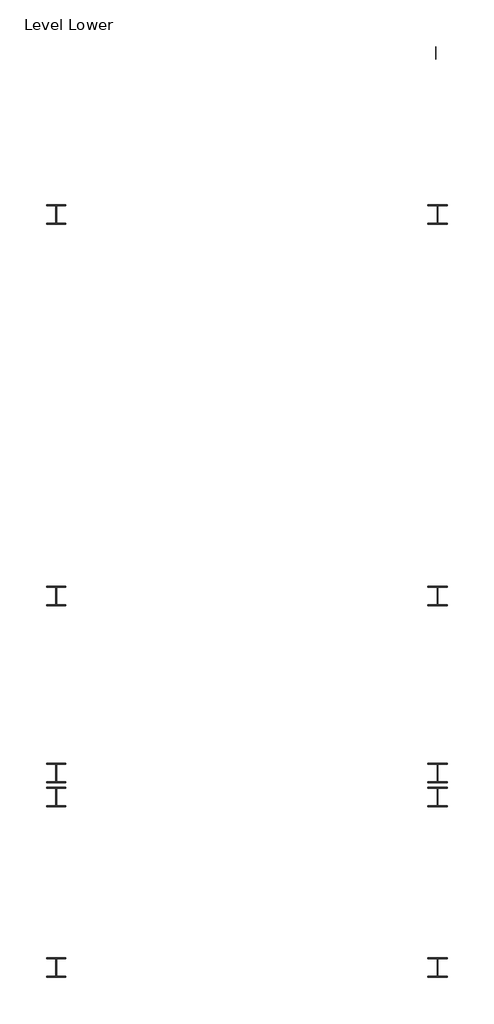
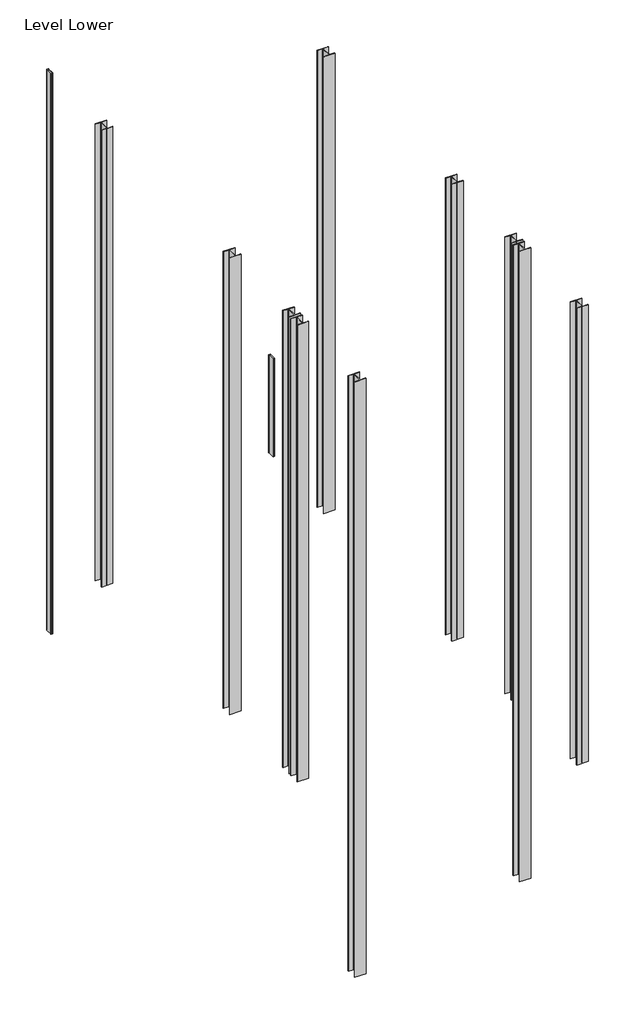
# One storey: 12 columns.
"""IFC4 building model written with IfcOpenShell, lengths in millimetres."""

import ifcopenshell
import ifcopenshell.guid

model = None  # the IFC model being written
_history = None  # IfcOwnerHistory: only IFC2X3 demands one
_inside = {}  # id of a spatial element -> (the spatial element, [elements in it])
_under = {}  # id of a project, library or spatial element -> (it, [spatial elements below it])
_declared = {}  # id of a project -> (the project, [libraries it declares])
_typed = {}  # id of a type object -> (the type object, [elements of that type])
_made_of = {}  # id of a material, layer set ... -> (it, [elements and type objects made of it])


def new_model(schema):
    """Start an empty IFC model of exactly this schema.

    Asked for "IFC4X3", IfcOpenShell would pick the latest addendum, in which some entities
    have other attributes; the version numbers below select the first issue.
    IFC2X3 requires an IfcOwnerHistory on every rooted entity: one is made here for all.
    """
    global model, _history
    if schema == "IFC4X3":
        model = ifcopenshell.file(schema_version=(4, 3, 0, 0))
    else:
        model = ifcopenshell.file(schema=schema)
    _inside.clear()
    _under.clear()
    _declared.clear()
    _typed.clear()
    _made_of.clear()
    _history = None
    if model.schema == "IFC2X3":
        org = make("IfcOrganization", Name="unknown")
        user = make(
            "IfcPersonAndOrganization",
            ThePerson=make("IfcPerson", FamilyName="unknown"),
            TheOrganization=org,
        )
        app = make(
            "IfcApplication",
            ApplicationDeveloper=org,
            Version="unknown",
            ApplicationFullName="unknown",
            ApplicationIdentifier="unknown",
        )
        _history = make(
            "IfcOwnerHistory",
            OwningUser=user,
            OwningApplication=app,
            ChangeAction="ADDED",
            CreationDate=0,
        )
    return model


def make(cls, **values):
    """One entity of the class cls with the attributes given. An attribute that is None is left unset."""
    return model.create_entity(
        cls, **{name: value for name, value in values.items() if value is not None}
    )


def rooted(cls, **values):
    """An entity with a GlobalId (a new one), such as an element, a storey or a relation."""
    return make(cls, GlobalId=ifcopenshell.guid.new(), OwnerHistory=_history, **values)


def si_unit(unit_type, name, prefix=None):
    """IfcSIUnit, for example si_unit("LENGTHUNIT", "METRE", prefix="MILLI")."""
    return make("IfcSIUnit", UnitType=unit_type, Prefix=prefix, Name=name)


def assignment(units):
    """IfcUnitAssignment: the units of a project."""
    return None if units is None else make("IfcUnitAssignment", Units=units)


def point(xyz):
    """IfcCartesianPoint."""
    return None if xyz is None else make("IfcCartesianPoint", Coordinates=xyz)


def direction(xyz):
    """IfcDirection."""
    return None if xyz is None else make("IfcDirection", DirectionRatios=xyz)


def frame(location, z_axis=None, x_axis=None):
    """IfcAxis2Placement3D, a coordinate frame: its origin and axes. An axis left out is left unset."""
    return make(
        "IfcAxis2Placement3D",
        Location=point(location),
        Axis=direction(z_axis),
        RefDirection=direction(x_axis),
    )


def frame_2d(location, x_axis=None):
    """IfcAxis2Placement2D, a coordinate frame in the plane: its origin and x axis."""
    return make(
        "IfcAxis2Placement2D", Location=point(location), RefDirection=direction(x_axis)
    )


def origin():
    """The frame at (0, 0, 0) with its axes left unset."""
    return frame((0.0, 0.0, 0.0))


def place(relative_to, where):
    """IfcLocalPlacement: puts the frame where relative to a parent placement (None: the world)."""
    return make(
        "IfcLocalPlacement", PlacementRelTo=relative_to, RelativePlacement=where
    )


def context(
    kind, dimensions, precision=None, world=None, true_north=None, identifier=None
):
    """IfcGeometricRepresentationContext, for example the 3D "Model" context."""
    return make(
        "IfcGeometricRepresentationContext",
        ContextIdentifier=identifier,
        ContextType=kind,
        CoordinateSpaceDimension=dimensions,
        Precision=precision,
        WorldCoordinateSystem=world,
        TrueNorth=true_north,
    )


def project(units=None, contexts=None):
    """IfcProject with its units and contexts."""
    return rooted(
        "IfcProject",
        Name="project",
        RepresentationContexts=contexts,
        UnitsInContext=assignment(units),
    )


def spatial(cls, under=None, at=None, **own):
    """A site, building, storey or space (cls), placed at a placement, below another one or the project."""
    s = rooted(cls, ObjectPlacement=at, **own)
    if under is not None:
        _under.setdefault(under.id(), (under, []))[1].append(s)
    return s


def polyline(points):
    """IfcPolyline through the points."""
    return make("IfcPolyline", Points=[point(p) for p in points])


def circle_curve(where, radius):
    """IfcCircle in the frame where."""
    return make("IfcCircle", Position=where, Radius=radius)


def trimmed(basis, trim1, trim2, sense, master):
    """IfcTrimmedCurve: the piece of a basis curve between two trims."""
    return make(
        "IfcTrimmedCurve",
        BasisCurve=basis,
        Trim1=trim1,
        Trim2=trim2,
        SenseAgreement=sense,
        MasterRepresentation=master,
    )


def segment(curve, same_sense, transition):
    """IfcCompositeCurveSegment."""
    return make(
        "IfcCompositeCurveSegment",
        Transition=transition,
        SameSense=same_sense,
        ParentCurve=curve,
    )


def composite_curve(segments, self_intersect=None):
    """IfcCompositeCurve: segments joined end to end."""
    return make("IfcCompositeCurve", Segments=segments, SelfIntersect=self_intersect)


def outline(outer, holes=None, kind="AREA"):
    """IfcArbitraryClosedProfileDef: a profile drawn as a closed curve; with holes, ...WithVoids."""
    if holes is None:
        return make("IfcArbitraryClosedProfileDef", ProfileType=kind, OuterCurve=outer)
    return make(
        "IfcArbitraryProfileDefWithVoids",
        ProfileType=kind,
        OuterCurve=outer,
        InnerCurves=holes,
    )


def extrude(swept, where, along, depth):
    """IfcExtrudedAreaSolid: the profile swept, set in the frame where, extruded along a direction by depth."""
    return make(
        "IfcExtrudedAreaSolid",
        SweptArea=swept,
        Position=where,
        ExtrudedDirection=direction(along),
        Depth=depth,
    )


def shape(context_of_items, identifier, shape_type, items):
    """IfcShapeRepresentation: the items that make up one representation, for example the "Body"."""
    return make(
        "IfcShapeRepresentation",
        ContextOfItems=context_of_items,
        RepresentationIdentifier=identifier,
        RepresentationType=shape_type,
        Items=items,
    )


def source(mapping_origin, context_of_items, identifier, shape_type, items):
    """IfcRepresentationMap: a shape defined once, which mapped items show again and again."""
    return make(
        "IfcRepresentationMap",
        MappingOrigin=mapping_origin,
        MappedRepresentation=shape(context_of_items, identifier, shape_type, items),
    )


def transform(
    local_origin,
    x_axis=None,
    y_axis=None,
    z_axis=None,
    scale=None,
    scale2=None,
    scale3=None,
    uniform=True,
):
    """IfcCartesianTransformationOperator3D, or its non-uniform kind. x_axis, y_axis, z_axis: its Axis1, 2, 3."""
    if uniform:
        return make(
            "IfcCartesianTransformationOperator3D",
            Axis1=direction(x_axis),
            Axis2=direction(y_axis),
            LocalOrigin=point(local_origin),
            Scale=scale,
            Axis3=direction(z_axis),
        )
    return make(
        "IfcCartesianTransformationOperator3DnonUniform",
        Axis1=direction(x_axis),
        Axis2=direction(y_axis),
        LocalOrigin=point(local_origin),
        Scale=scale,
        Axis3=direction(z_axis),
        Scale2=scale2,
        Scale3=scale3,
    )


def mapped(mapping_source, mapping_target):
    """IfcMappedItem: shows the shape of a source again, moved by a transform."""
    return make(
        "IfcMappedItem", MappingSource=mapping_source, MappingTarget=mapping_target
    )


def made_of(thing, what):
    """Note that an element or type object is made of a material, layer set ...; save() writes the relation."""
    if what is not None:
        _made_of.setdefault(what.id(), (what, []))[1].append(thing)
    return thing


def element(
    cls,
    number,
    at=None,
    inside=None,
    cuts=None,
    type_object=None,
    material=None,
    context=None,
    identifier="Body",
    shape_type=None,
    held_by="IfcProductDefinitionShape",
    body=None,
    shapes=None,
    **own,
):
    """One element of the class cls, such as IfcWall. Its Tag is "e" and its number.

    at: its placement. inside: the storey or other place that contains it. cuts: it is an
    opening in that element (IfcRelVoidsElement). A single representation is given by context,
    identifier, shape_type and body (its items); several are given by shapes. held_by: the class
    of the entity that holds the representations. save() writes the other relations.
    """
    e = rooted(cls, Tag="e%d" % number, ObjectPlacement=at, **own)
    if body is not None:
        shapes = [shape(context, identifier, shape_type, body)]
    if shapes is not None:
        e.Representation = make(held_by, Representations=shapes)
    if inside is not None:
        _inside.setdefault(inside.id(), (inside, []))[1].append(e)
    if cuts is not None:
        rooted(
            "IfcRelVoidsElement", RelatingBuildingElement=cuts, RelatedOpeningElement=e
        )
    if type_object is not None:
        _typed.setdefault(type_object.id(), (type_object, []))[1].append(e)
    return made_of(e, material)


def aggregate(whole, parts):
    """IfcRelAggregates: a whole, such as a stair, and the parts it consists of."""
    return rooted("IfcRelAggregates", RelatingObject=whole, RelatedObjects=parts)


def save(model, path):
    """Write the relations noted so far, then the file.

    IfcRelAggregates (storeys below a building ...), IfcRelContainedInSpatialStructure (elements
    in a storey), IfcRelDefinesByType, IfcRelAssociatesMaterial and IfcRelDeclares: one each for
    every whole, place, type object, material and project.
    """
    for whole, parts in _under.values():
        aggregate(whole, parts)
    for where, things in _inside.values():
        rooted(
            "IfcRelContainedInSpatialStructure",
            RelatedElements=things,
            RelatingStructure=where,
        )
    for kind, things in _typed.values():
        rooted("IfcRelDefinesByType", RelatedObjects=things, RelatingType=kind)
    for what, things in _made_of.values():
        rooted("IfcRelAssociatesMaterial", RelatedObjects=things, RelatingMaterial=what)
    for by, libraries in _declared.values():
        rooted("IfcRelDeclares", RelatingContext=by, RelatedDefinitions=libraries)
    model.write(path)


def hss_hollow_structural_section_column_hss8x2x3_16_e82f30fd(model_context):
    return source(origin(), model_context, "Body", "SweptSolid", [
        extrude(outline(composite_curve([segment(trimmed(circle_curve(frame_2d((16.5608, 92.7608)), 8.8392), [point((16.5608, 101.6))], [point((25.4, 92.7608))], False, "CARTESIAN"), True, "CONTINUOUS"), segment(polyline([(25.4, 92.7608), (25.4, -92.7608)]), True, "CONTINUOUS"), segment(trimmed(circle_curve(frame_2d((16.5608, -92.7608)), 8.8392), [point((25.4, -92.7608))], [point((16.5608, -101.6))], False, "CARTESIAN"), True, "CONTINUOUS"), segment(polyline([(16.5608, -101.6), (-16.5608, -101.6)]), True, "CONTINUOUS"), segment(trimmed(circle_curve(frame_2d((-16.5608, -92.7608)), 8.8392), [point((-16.5608, -101.6))], [point((-25.4, -92.7608))], False, "CARTESIAN"), True, "CONTINUOUS"), segment(polyline([(-25.4, -92.7608), (-25.4, 92.7608)]), True, "CONTINUOUS"), segment(trimmed(circle_curve(frame_2d((-16.5608, 92.7608)), 8.8392), [point((-25.4, 92.7608))], [point((-16.5608, 101.6))], False, "CARTESIAN"), True, "CONTINUOUS"), segment(polyline([(-16.5608, 101.6), (16.5608, 101.6)]), True, "CONTINUOUS")], self_intersect=False), holes=[composite_curve([segment(polyline([(16.5608, 97.1804), (-16.5608, 97.1804)]), True, "CONTINUOUS"), segment(trimmed(circle_curve(frame_2d((-16.5608, 92.7608)), 4.4196), [point((-16.5608, 97.1804))], [point((-20.9804, 92.7608))], True, "CARTESIAN"), True, "CONTINUOUS"), segment(polyline([(-20.9804, 92.7608), (-20.9804, -92.7608)]), True, "CONTINUOUS"), segment(trimmed(circle_curve(frame_2d((-16.5608, -92.7608)), 4.4196), [point((-20.9804, -92.7608))], [point((-16.5608, -97.1804))], True, "CARTESIAN"), True, "CONTINUOUS"), segment(polyline([(-16.5608, -97.1804), (16.5608, -97.1804)]), True, "CONTINUOUS"), segment(trimmed(circle_curve(frame_2d((16.5608, -92.7608)), 4.4196), [point((16.5608, -97.1804))], [point((20.9804, -92.7608))], True, "CARTESIAN"), True, "CONTINUOUS"), segment(polyline([(20.9804, -92.7608), (20.9804, 92.7608)]), True, "CONTINUOUS"), segment(trimmed(circle_curve(frame_2d((16.5608, 92.7608)), 4.4196), [point((20.9804, 92.7608))], [point((16.5608, 97.1804))], True, "CARTESIAN"), True, "CONTINUOUS")], self_intersect=False)]), frame((0.0, 0.0, -594.0), z_axis=(0.0, 0.0, 1.0), x_axis=(1.0, 0.0, 0.0)), (0.0, 0.0, 1.0), 2793.0),
    ])


def hss_hollow_structural_section_column_hss8x2x3_16_37e330f9(model_context):
    return source(origin(), model_context, "Body", "SweptSolid", [
        extrude(outline(composite_curve([segment(trimmed(circle_curve(frame_2d((16.5608, 92.7608)), 8.8392), [point((16.5608, 101.6))], [point((25.4, 92.7608))], False, "CARTESIAN"), True, "CONTINUOUS"), segment(polyline([(25.4, 92.7608), (25.4, -92.7608)]), True, "CONTINUOUS"), segment(trimmed(circle_curve(frame_2d((16.5608, -92.7608)), 8.8392), [point((25.4, -92.7608))], [point((16.5608, -101.6))], False, "CARTESIAN"), True, "CONTINUOUS"), segment(polyline([(16.5608, -101.6), (-16.5608, -101.6)]), True, "CONTINUOUS"), segment(trimmed(circle_curve(frame_2d((-16.5608, -92.7608)), 8.8392), [point((-16.5608, -101.6))], [point((-25.4, -92.7608))], False, "CARTESIAN"), True, "CONTINUOUS"), segment(polyline([(-25.4, -92.7608), (-25.4, 92.7608)]), True, "CONTINUOUS"), segment(trimmed(circle_curve(frame_2d((-16.5608, 92.7608)), 8.8392), [point((-25.4, 92.7608))], [point((-16.5608, 101.6))], False, "CARTESIAN"), True, "CONTINUOUS"), segment(polyline([(-16.5608, 101.6), (16.5608, 101.6)]), True, "CONTINUOUS")], self_intersect=False), holes=[composite_curve([segment(polyline([(16.5608, 97.1804), (-16.5608, 97.1804)]), True, "CONTINUOUS"), segment(trimmed(circle_curve(frame_2d((-16.5608, 92.7608)), 4.4196), [point((-16.5608, 97.1804))], [point((-20.9804, 92.7608))], True, "CARTESIAN"), True, "CONTINUOUS"), segment(polyline([(-20.9804, 92.7608), (-20.9804, -92.7608)]), True, "CONTINUOUS"), segment(trimmed(circle_curve(frame_2d((-16.5608, -92.7608)), 4.4196), [point((-20.9804, -92.7608))], [point((-16.5608, -97.1804))], True, "CARTESIAN"), True, "CONTINUOUS"), segment(polyline([(-16.5608, -97.1804), (16.5608, -97.1804)]), True, "CONTINUOUS"), segment(trimmed(circle_curve(frame_2d((16.5608, -92.7608)), 4.4196), [point((16.5608, -97.1804))], [point((20.9804, -92.7608))], True, "CARTESIAN"), True, "CONTINUOUS"), segment(polyline([(20.9804, -92.7608), (20.9804, 92.7608)]), True, "CONTINUOUS"), segment(trimmed(circle_curve(frame_2d((16.5608, 92.7608)), 4.4196), [point((20.9804, 92.7608))], [point((16.5608, 97.1804))], True, "CARTESIAN"), True, "CONTINUOUS")], self_intersect=False)]), frame((0.0, 0.0, -3550.0), z_axis=(0.0, 0.0, 1.0), x_axis=(1.0, 0.0, 0.0)), (0.0, 0.0, 1.0), 15989.0),
    ])


def uc_universal_columns_column_uc305x305x97_fcd1f718(model_context):
    return source(origin(), model_context, "Body", "SweptSolid", [
        extrude(outline(composite_curve([segment(polyline([(152.65, 153.95), (152.65, 138.55), (20.15, 138.55)]), True, "CONTINUOUS"), segment(trimmed(circle_curve(frame_2d((20.15, 123.35)), 15.2), [point((20.15, 138.55))], [point((4.95, 123.35))], True, "CARTESIAN"), True, "CONTINUOUS"), segment(polyline([(4.95, 123.35), (4.95, -123.35)]), True, "CONTINUOUS"), segment(trimmed(circle_curve(frame_2d((20.15, -123.35)), 15.2), [point((4.95, -123.35))], [point((20.15, -138.55))], True, "CARTESIAN"), True, "CONTINUOUS"), segment(polyline([(20.15, -138.55), (152.65, -138.55), (152.65, -153.95), (-152.65, -153.95), (-152.65, -138.55), (-20.15, -138.55)]), True, "CONTINUOUS"), segment(trimmed(circle_curve(frame_2d((-20.15, -123.35)), 15.2), [point((-20.15, -138.55))], [point((-4.95, -123.35))], True, "CARTESIAN"), True, "CONTINUOUS"), segment(polyline([(-4.95, -123.35), (-4.95, 123.35)]), True, "CONTINUOUS"), segment(trimmed(circle_curve(frame_2d((-20.15, 123.35)), 15.2), [point((-4.95, 123.35))], [point((-20.15, 138.55))], True, "CARTESIAN"), True, "CONTINUOUS"), segment(polyline([(-20.15, 138.55), (-152.65, 138.55), (-152.65, 153.95), (152.65, 153.95)]), True, "CONTINUOUS")], self_intersect=False)), frame((0.0, 0.0, -594.0), z_axis=(0.0, 0.0, 1.0), x_axis=(1.0, 0.0, 0.0)), (0.0, 0.0, 1.0), 13033.0),
    ])


def uc_universal_columns_column_uc305x305x97_02d5a26a(model_context):
    return source(origin(), model_context, "Body", "SweptSolid", [
        extrude(outline(composite_curve([segment(polyline([(152.65, 153.95), (152.65, 138.55), (20.15, 138.55)]), True, "CONTINUOUS"), segment(trimmed(circle_curve(frame_2d((20.15, 123.35)), 15.2), [point((20.15, 138.55))], [point((4.95, 123.35))], True, "CARTESIAN"), True, "CONTINUOUS"), segment(polyline([(4.95, 123.35), (4.95, -123.35)]), True, "CONTINUOUS"), segment(trimmed(circle_curve(frame_2d((20.15, -123.35)), 15.2), [point((4.95, -123.35))], [point((20.15, -138.55))], True, "CARTESIAN"), True, "CONTINUOUS"), segment(polyline([(20.15, -138.55), (152.65, -138.55), (152.65, -153.95), (-152.65, -153.95), (-152.65, -138.55), (-20.15, -138.55)]), True, "CONTINUOUS"), segment(trimmed(circle_curve(frame_2d((-20.15, -123.35)), 15.2), [point((-20.15, -138.55))], [point((-4.95, -123.35))], True, "CARTESIAN"), True, "CONTINUOUS"), segment(polyline([(-4.95, -123.35), (-4.95, 123.35)]), True, "CONTINUOUS"), segment(trimmed(circle_curve(frame_2d((-20.15, 123.35)), 15.2), [point((-4.95, 123.35))], [point((-20.15, 138.55))], True, "CARTESIAN"), True, "CONTINUOUS"), segment(polyline([(-20.15, 138.55), (-152.65, 138.55), (-152.65, 153.95), (152.65, 153.95)]), True, "CONTINUOUS")], self_intersect=False)), frame((0.0, 0.0, -4550.0), z_axis=(0.0, 0.0, 1.0), x_axis=(1.0, 0.0, 0.0)), (0.0, 0.0, 1.0), 16989.0),
    ])


def uc_universal_columns_column_uc305x305x97_e2fb10fc(model_context):
    return source(origin(), model_context, "Body", "SweptSolid", [
        extrude(outline(composite_curve([segment(polyline([(152.65, 153.95), (152.65, 138.55), (20.15, 138.55)]), True, "CONTINUOUS"), segment(trimmed(circle_curve(frame_2d((20.15, 123.35)), 15.2), [point((20.15, 138.55))], [point((4.95, 123.35))], True, "CARTESIAN"), True, "CONTINUOUS"), segment(polyline([(4.95, 123.35), (4.95, -123.35)]), True, "CONTINUOUS"), segment(trimmed(circle_curve(frame_2d((20.15, -123.35)), 15.2), [point((4.95, -123.35))], [point((20.15, -138.55))], True, "CARTESIAN"), True, "CONTINUOUS"), segment(polyline([(20.15, -138.55), (152.65, -138.55), (152.65, -153.95), (-152.65, -153.95), (-152.65, -138.55), (-20.15, -138.55)]), True, "CONTINUOUS"), segment(trimmed(circle_curve(frame_2d((-20.15, -123.35)), 15.2), [point((-20.15, -138.55))], [point((-4.95, -123.35))], True, "CARTESIAN"), True, "CONTINUOUS"), segment(polyline([(-4.95, -123.35), (-4.95, 123.35)]), True, "CONTINUOUS"), segment(trimmed(circle_curve(frame_2d((-20.15, 123.35)), 15.2), [point((-4.95, 123.35))], [point((-20.15, 138.55))], True, "CARTESIAN"), True, "CONTINUOUS"), segment(polyline([(-20.15, 138.55), (-152.65, 138.55), (-152.65, 153.95), (152.65, 153.95)]), True, "CONTINUOUS")], self_intersect=False)), frame((0.0, 0.0, -5550.0), z_axis=(0.0, 0.0, 1.0), x_axis=(1.0, 0.0, 0.0)), (0.0, 0.0, 1.0), 17989.0),
    ])


model = new_model("IFC4")

# Units and contexts
model_context = context("Model", 3, world=origin())
ifc_project = project(units=[si_unit("LENGTHUNIT", "METRE", prefix="MILLI")], contexts=[model_context])

# Site, building, storey
site = spatial("IfcSite", under=ifc_project)
building = spatial("IfcBuilding", under=site)
storey = spatial("IfcBuildingStorey", under=building, Name="Level Lower", Elevation=-550.0)

# Columns
placement = place(None, origin())
hss_hollow_structural_section_column_hss8x2x3_16_shape = hss_hollow_structural_section_column_hss8x2x3_16_e82f30fd(model_context)
element("IfcColumn", 1, ObjectType="HSS-Hollow Structural Section-Column : HSS8X2X3/16", at=placement, inside=storey, context=model_context, shape_type="MappedRepresentation", body=[
    mapped(hss_hollow_structural_section_column_hss8x2x3_16_shape, transform((13061.9315174, -3661.5939786, 0.0), x_axis=(1.0, 0.0, 0.0), y_axis=(0.0, 1.0, 0.0), z_axis=(0.0, 0.0, 1.0))),
])
hss_hollow_structural_section_column_hss8x2x3_16_2_shape = hss_hollow_structural_section_column_hss8x2x3_16_37e330f9(model_context)
element("IfcColumn", 2, ObjectType="HSS-Hollow Structural Section-Column : HSS8X2X3/16", at=placement, inside=storey, context=model_context, shape_type="MappedRepresentation", body=[
    mapped(hss_hollow_structural_section_column_hss8x2x3_16_2_shape, transform((7061.9315174, -3661.5939786, 0.0), x_axis=(1.0, 0.0, 0.0), y_axis=(0.0, 1.0, 0.0), z_axis=(0.0, 0.0, 1.0))),
])
uc_universal_columns_column_uc305x305x97_shape = uc_universal_columns_column_uc305x305x97_fcd1f718(model_context)
element("IfcColumn", 3, ObjectType="UC-Universal Columns-Column : UC305x305x97", at=placement, inside=storey, context=model_context, shape_type="MappedRepresentation", body=[
    mapped(uc_universal_columns_column_uc305x305x97_shape, transform((7061.9315174, -15361.5939786, 0.0), x_axis=(1.0, 0.0, 0.0), y_axis=(0.0, 1.0, 0.0), z_axis=(0.0, 0.0, 1.0))),
])
element("IfcColumn", 4, ObjectType="UC-Universal Columns-Column : UC305x305x97", at=placement, inside=storey, context=model_context, shape_type="MappedRepresentation", body=[
    mapped(uc_universal_columns_column_uc305x305x97_shape, transform((7061.9315174, -14981.5939786, 0.0), x_axis=(1.0, 0.0, 0.0), y_axis=(0.0, 1.0, 0.0), z_axis=(0.0, 0.0, 1.0))),
])
element("IfcColumn", 5, ObjectType="UC-Universal Columns-Column : UC305x305x97", at=placement, inside=storey, context=model_context, shape_type="MappedRepresentation", body=[
    mapped(uc_universal_columns_column_uc305x305x97_shape, transform((7061.9315174, -12201.5939786, 0.0), x_axis=(1.0, 0.0, 0.0), y_axis=(0.0, 1.0, 0.0), z_axis=(0.0, 0.0, 1.0))),
])
element("IfcColumn", 6, ObjectType="UC-Universal Columns-Column : UC305x305x97", at=placement, inside=storey, context=model_context, shape_type="MappedRepresentation", body=[
    mapped(uc_universal_columns_column_uc305x305x97_shape, transform((7061.9315174, -6201.5939786, 0.0), x_axis=(1.0, 0.0, 0.0), y_axis=(0.0, 1.0, 0.0), z_axis=(0.0, 0.0, 1.0))),
])
element("IfcColumn", 7, ObjectType="UC-Universal Columns-Column : UC305x305x97", at=placement, inside=storey, context=model_context, shape_type="MappedRepresentation", body=[
    mapped(uc_universal_columns_column_uc305x305x97_shape, transform((13061.9315174, -14981.5939786, 0.0), x_axis=(1.0, 0.0, 0.0), y_axis=(0.0, 1.0, 0.0), z_axis=(0.0, 0.0, 1.0))),
])
element("IfcColumn", 8, ObjectType="UC-Universal Columns-Column : UC305x305x97", at=placement, inside=storey, context=model_context, shape_type="MappedRepresentation", body=[
    mapped(uc_universal_columns_column_uc305x305x97_shape, transform((13061.9315174, -12201.5939786, 0.0), x_axis=(1.0, 0.0, 0.0), y_axis=(0.0, 1.0, 0.0), z_axis=(0.0, 0.0, 1.0))),
])
element("IfcColumn", 9, ObjectType="UC-Universal Columns-Column : UC305x305x97", at=placement, inside=storey, context=model_context, shape_type="MappedRepresentation", body=[
    mapped(uc_universal_columns_column_uc305x305x97_shape, transform((13061.9315174, -6201.5939786, 0.0), x_axis=(1.0, 0.0, 0.0), y_axis=(0.0, 1.0, 0.0), z_axis=(0.0, 0.0, 1.0))),
])
element("IfcColumn", 10, ObjectType="UC-Universal Columns-Column : UC305x305x97", at=placement, inside=storey, context=model_context, shape_type="MappedRepresentation", body=[
    mapped(uc_universal_columns_column_uc305x305x97_shape, transform((13061.9315174, -18041.5939786, 0.0), x_axis=(1.0, 0.0, 0.0), y_axis=(0.0, 1.0, 0.0), z_axis=(0.0, 0.0, 1.0))),
])
uc_universal_columns_column_uc305x305x97_2_shape = uc_universal_columns_column_uc305x305x97_02d5a26a(model_context)
element("IfcColumn", 11, ObjectType="UC-Universal Columns-Column : UC305x305x97", at=placement, inside=storey, context=model_context, shape_type="MappedRepresentation", body=[
    mapped(uc_universal_columns_column_uc305x305x97_2_shape, transform((7061.9315174, -18041.5939786, 0.0), x_axis=(1.0, 0.0, 0.0), y_axis=(0.0, 1.0, 0.0), z_axis=(0.0, 0.0, 1.0))),
])
uc_universal_columns_column_uc305x305x97_3_shape = uc_universal_columns_column_uc305x305x97_e2fb10fc(model_context)
element("IfcColumn", 12, ObjectType="UC-Universal Columns-Column : UC305x305x97", at=placement, inside=storey, context=model_context, shape_type="MappedRepresentation", body=[
    mapped(uc_universal_columns_column_uc305x305x97_3_shape, transform((13061.9315174, -15361.5939786, 0.0), x_axis=(1.0, 0.0, 0.0), y_axis=(0.0, 1.0, 0.0), z_axis=(0.0, 0.0, 1.0))),
])

save(model, "model.ifc")

# Revit data of these elements
# Type "HSS-Hollow Structural Section-Column : HSS8X2X3/16"
#   Assembly Code = "B10"
#   Shape = "Rect."
#   Cost = 1
#   W = 12
#   Ht = 203.2 mm
#   b = 50.8 mm
#   kr = 8.839 mm
#   t = 4.42 mm
#   A = 0.00211612 m²
#   Structural Material [instance default] = Steel ASTM A500, Grade B, Rectangular and Square
# Type "UC-Universal Columns-Column : UC305x305x97"
#   Section Name Key = "UC305x305x97"
#   Cost = 2
#   Width = 30.53 cm
#   Web Thickness = 0.99 cm
#   Web Fillet = 1.52 cm
#   Warping Constant = 1560000.0 cm⁶
#   Torsional Moment of Inertia = 91.20 cm⁴
#   Section Area = 123.0 cm²
#   Plastic Modulus weak axis = 726.0 cm³
#   Plastic Modulus strong axis = 1592.0 cm³
#   Nominal Weight = 96.8996 kgf/m
#   Moment of Inertia weak axis = 7308.00 cm⁴
#   Moment of Inertia strong axis = 22249.00 cm⁴
#   Height = 30.79 cm
#   Flange Thickness = 1.54 cm
#   Elastic Modulus weak axis = 479.0 cm³
#   Elastic Modulus strong axis = 1445.0 cm³
#   Centroid Vertical = 15.395 cm
#   Centroid Horizontal = 15.265 cm
#   Bolt Spacing = 14.0 cm
#   Structural Material [instance default] = Metal - Steel 43-275
#   Type Comments = ""
#   Assembly Code = ""
# Elements 1, 2 (IfcColumn, "HSS-Hollow Structural Section-Column : HSS8X2X3/16")
#   Structural Material = Metal - Steel 43-275
#   Phase Created = New Construction
#   Materials on its faces: "Metal - Steel 43-275"
# Elements 3, 4, 5, 6, 7, 8, 9, 10, 11, 12 (IfcColumn, "UC-Universal Columns-Column : UC305x305x97")
#   Structural Material = Metal - Steel 43-275
#   Phase Created = New Construction
#   Materials on its faces: "Metal - Steel 43-275"
# Materials
#   "Steel ASTM A500, Grade B, Rectangular and Square": class "Metal", colour RGB 199 199 199, transparency 0, Description = "Carbon steel", Cost = 0
#   "Metal - Steel 43-275": class "Metal", colour RGB 247 247 247, transparency 0, Cost = 0
